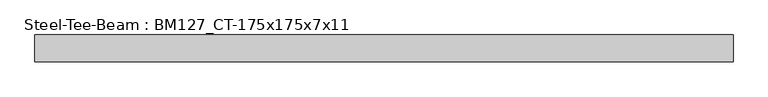
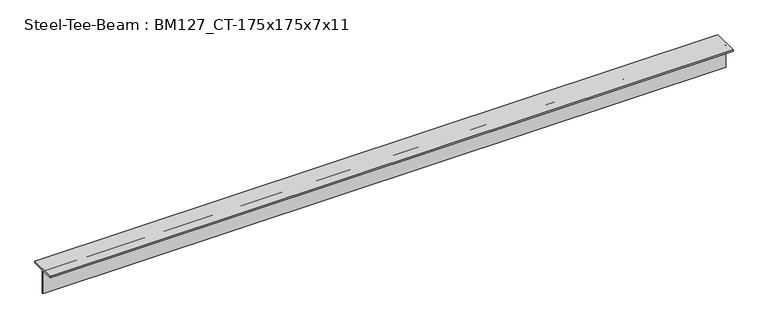
"""IFC4 building model written with IfcOpenShell, lengths in millimetres: beam geometry, Steel-Tee-Beam : BM127_CT-175x175x7x11."""

import ifcopenshell
import ifcopenshell.guid

model = None  # the IFC model being written
_history = None  # IfcOwnerHistory: only IFC2X3 demands one
_inside = {}  # id of a spatial element -> (the spatial element, [elements in it])
_under = {}  # id of a project, library or spatial element -> (it, [spatial elements below it])
_declared = {}  # id of a project -> (the project, [libraries it declares])
_typed = {}  # id of a type object -> (the type object, [elements of that type])
_made_of = {}  # id of a material, layer set ... -> (it, [elements and type objects made of it])


def new_model(schema):
    """Start an empty IFC model of exactly this schema.

    Asked for "IFC4X3", IfcOpenShell would pick the latest addendum, in which some entities
    have other attributes; the version numbers below select the first issue.
    IFC2X3 requires an IfcOwnerHistory on every rooted entity: one is made here for all.
    """
    global model, _history
    if schema == "IFC4X3":
        model = ifcopenshell.file(schema_version=(4, 3, 0, 0))
    else:
        model = ifcopenshell.file(schema=schema)
    _inside.clear()
    _under.clear()
    _declared.clear()
    _typed.clear()
    _made_of.clear()
    _history = None
    if model.schema == "IFC2X3":
        org = make("IfcOrganization", Name="unknown")
        user = make(
            "IfcPersonAndOrganization",
            ThePerson=make("IfcPerson", FamilyName="unknown"),
            TheOrganization=org,
        )
        app = make(
            "IfcApplication",
            ApplicationDeveloper=org,
            Version="unknown",
            ApplicationFullName="unknown",
            ApplicationIdentifier="unknown",
        )
        _history = make(
            "IfcOwnerHistory",
            OwningUser=user,
            OwningApplication=app,
            ChangeAction="ADDED",
            CreationDate=0,
        )
    return model


def make(cls, **values):
    """One entity of the class cls with the attributes given. An attribute that is None is left unset."""
    return model.create_entity(
        cls, **{name: value for name, value in values.items() if value is not None}
    )


def rooted(cls, **values):
    """An entity with a GlobalId (a new one), such as an element, a storey or a relation."""
    return make(cls, GlobalId=ifcopenshell.guid.new(), OwnerHistory=_history, **values)


def si_unit(unit_type, name, prefix=None):
    """IfcSIUnit, for example si_unit("LENGTHUNIT", "METRE", prefix="MILLI")."""
    return make("IfcSIUnit", UnitType=unit_type, Prefix=prefix, Name=name)


def assignment(units):
    """IfcUnitAssignment: the units of a project."""
    return None if units is None else make("IfcUnitAssignment", Units=units)


def point(xyz):
    """IfcCartesianPoint."""
    return None if xyz is None else make("IfcCartesianPoint", Coordinates=xyz)


def direction(xyz):
    """IfcDirection."""
    return None if xyz is None else make("IfcDirection", DirectionRatios=xyz)


def frame(location, z_axis=None, x_axis=None):
    """IfcAxis2Placement3D, a coordinate frame: its origin and axes. An axis left out is left unset."""
    return make(
        "IfcAxis2Placement3D",
        Location=point(location),
        Axis=direction(z_axis),
        RefDirection=direction(x_axis),
    )


def frame_2d(location, x_axis=None):
    """IfcAxis2Placement2D, a coordinate frame in the plane: its origin and x axis."""
    return make(
        "IfcAxis2Placement2D", Location=point(location), RefDirection=direction(x_axis)
    )


def origin():
    """The frame at (0, 0, 0) with its axes left unset."""
    return frame((0.0, 0.0, 0.0))


def place(relative_to, where):
    """IfcLocalPlacement: puts the frame where relative to a parent placement (None: the world)."""
    return make(
        "IfcLocalPlacement", PlacementRelTo=relative_to, RelativePlacement=where
    )


def context(
    kind, dimensions, precision=None, world=None, true_north=None, identifier=None
):
    """IfcGeometricRepresentationContext, for example the 3D "Model" context."""
    return make(
        "IfcGeometricRepresentationContext",
        ContextIdentifier=identifier,
        ContextType=kind,
        CoordinateSpaceDimension=dimensions,
        Precision=precision,
        WorldCoordinateSystem=world,
        TrueNorth=true_north,
    )


def project(units=None, contexts=None):
    """IfcProject with its units and contexts."""
    return rooted(
        "IfcProject",
        Name="project",
        RepresentationContexts=contexts,
        UnitsInContext=assignment(units),
    )


def spatial(cls, under=None, at=None, **own):
    """A site, building, storey or space (cls), placed at a placement, below another one or the project."""
    s = rooted(cls, ObjectPlacement=at, **own)
    if under is not None:
        _under.setdefault(under.id(), (under, []))[1].append(s)
    return s


def polyline(points):
    """IfcPolyline through the points."""
    return make("IfcPolyline", Points=[point(p) for p in points])


def circle_curve(where, radius):
    """IfcCircle in the frame where."""
    return make("IfcCircle", Position=where, Radius=radius)


def trimmed(basis, trim1, trim2, sense, master):
    """IfcTrimmedCurve: the piece of a basis curve between two trims."""
    return make(
        "IfcTrimmedCurve",
        BasisCurve=basis,
        Trim1=trim1,
        Trim2=trim2,
        SenseAgreement=sense,
        MasterRepresentation=master,
    )


def segment(curve, same_sense, transition):
    """IfcCompositeCurveSegment."""
    return make(
        "IfcCompositeCurveSegment",
        Transition=transition,
        SameSense=same_sense,
        ParentCurve=curve,
    )


def composite_curve(segments, self_intersect=None):
    """IfcCompositeCurve: segments joined end to end."""
    return make("IfcCompositeCurve", Segments=segments, SelfIntersect=self_intersect)


def outline(outer, holes=None, kind="AREA"):
    """IfcArbitraryClosedProfileDef: a profile drawn as a closed curve; with holes, ...WithVoids."""
    if holes is None:
        return make("IfcArbitraryClosedProfileDef", ProfileType=kind, OuterCurve=outer)
    return make(
        "IfcArbitraryProfileDefWithVoids",
        ProfileType=kind,
        OuterCurve=outer,
        InnerCurves=holes,
    )


def extrude(swept, where, along, depth):
    """IfcExtrudedAreaSolid: the profile swept, set in the frame where, extruded along a direction by depth."""
    return make(
        "IfcExtrudedAreaSolid",
        SweptArea=swept,
        Position=where,
        ExtrudedDirection=direction(along),
        Depth=depth,
    )


def shape(context_of_items, identifier, shape_type, items):
    """IfcShapeRepresentation: the items that make up one representation, for example the "Body"."""
    return make(
        "IfcShapeRepresentation",
        ContextOfItems=context_of_items,
        RepresentationIdentifier=identifier,
        RepresentationType=shape_type,
        Items=items,
    )


def source(mapping_origin, context_of_items, identifier, shape_type, items):
    """IfcRepresentationMap: a shape defined once, which mapped items show again and again."""
    return make(
        "IfcRepresentationMap",
        MappingOrigin=mapping_origin,
        MappedRepresentation=shape(context_of_items, identifier, shape_type, items),
    )


def transform(
    local_origin,
    x_axis=None,
    y_axis=None,
    z_axis=None,
    scale=None,
    scale2=None,
    scale3=None,
    uniform=True,
):
    """IfcCartesianTransformationOperator3D, or its non-uniform kind. x_axis, y_axis, z_axis: its Axis1, 2, 3."""
    if uniform:
        return make(
            "IfcCartesianTransformationOperator3D",
            Axis1=direction(x_axis),
            Axis2=direction(y_axis),
            LocalOrigin=point(local_origin),
            Scale=scale,
            Axis3=direction(z_axis),
        )
    return make(
        "IfcCartesianTransformationOperator3DnonUniform",
        Axis1=direction(x_axis),
        Axis2=direction(y_axis),
        LocalOrigin=point(local_origin),
        Scale=scale,
        Axis3=direction(z_axis),
        Scale2=scale2,
        Scale3=scale3,
    )


def mapped(mapping_source, mapping_target):
    """IfcMappedItem: shows the shape of a source again, moved by a transform."""
    return make(
        "IfcMappedItem", MappingSource=mapping_source, MappingTarget=mapping_target
    )


def made_of(thing, what):
    """Note that an element or type object is made of a material, layer set ...; save() writes the relation."""
    if what is not None:
        _made_of.setdefault(what.id(), (what, []))[1].append(thing)
    return thing


def element(
    cls,
    number,
    at=None,
    inside=None,
    cuts=None,
    type_object=None,
    material=None,
    context=None,
    identifier="Body",
    shape_type=None,
    held_by="IfcProductDefinitionShape",
    body=None,
    shapes=None,
    **own,
):
    """One element of the class cls, such as IfcWall. Its Tag is "e" and its number.

    at: its placement. inside: the storey or other place that contains it. cuts: it is an
    opening in that element (IfcRelVoidsElement). A single representation is given by context,
    identifier, shape_type and body (its items); several are given by shapes. held_by: the class
    of the entity that holds the representations. save() writes the other relations.
    """
    e = rooted(cls, Tag="e%d" % number, ObjectPlacement=at, **own)
    if body is not None:
        shapes = [shape(context, identifier, shape_type, body)]
    if shapes is not None:
        e.Representation = make(held_by, Representations=shapes)
    if inside is not None:
        _inside.setdefault(inside.id(), (inside, []))[1].append(e)
    if cuts is not None:
        rooted(
            "IfcRelVoidsElement", RelatingBuildingElement=cuts, RelatedOpeningElement=e
        )
    if type_object is not None:
        _typed.setdefault(type_object.id(), (type_object, []))[1].append(e)
    return made_of(e, material)


def aggregate(whole, parts):
    """IfcRelAggregates: a whole, such as a stair, and the parts it consists of."""
    return rooted("IfcRelAggregates", RelatingObject=whole, RelatedObjects=parts)


def save(model, path):
    """Write the relations noted so far, then the file.

    IfcRelAggregates (storeys below a building ...), IfcRelContainedInSpatialStructure (elements
    in a storey), IfcRelDefinesByType, IfcRelAssociatesMaterial and IfcRelDeclares: one each for
    every whole, place, type object, material and project.
    """
    for whole, parts in _under.values():
        aggregate(whole, parts)
    for where, things in _inside.values():
        rooted(
            "IfcRelContainedInSpatialStructure",
            RelatedElements=things,
            RelatingStructure=where,
        )
    for kind, things in _typed.values():
        rooted("IfcRelDefinesByType", RelatedObjects=things, RelatingType=kind)
    for what, things in _made_of.values():
        rooted("IfcRelAssociatesMaterial", RelatedObjects=things, RelatingMaterial=what)
    for by, libraries in _declared.values():
        rooted("IfcRelDeclares", RelatingContext=by, RelatedDefinitions=libraries)
    model.write(path)


def steel_tee_beam_bm127_ct_175x175x7x11_df70e9a8(model_context):
    return source(origin(), model_context, "Body", "SweptSolid", [
        extrude(outline(composite_curve([segment(polyline([(87.5, 87.5), (87.5, 76.5), (17.5, 76.5)]), True, "CONTINUOUS"), segment(trimmed(circle_curve(frame_2d((17.5, 62.5)), 14.0), [point((17.5, 76.5))], [point((3.5, 62.5))], True, "CARTESIAN"), True, "CONTINUOUS"), segment(polyline([(3.5, 62.5), (3.5, -87.5), (-3.5, -87.5), (-3.5, 62.5)]), True, "CONTINUOUS"), segment(trimmed(circle_curve(frame_2d((-17.5, 62.5)), 14.0), [point((-3.5, 62.5))], [point((-17.5, 76.5))], True, "CARTESIAN"), True, "CONTINUOUS"), segment(polyline([(-17.5, 76.5), (-87.5, 76.5), (-87.5, 87.5), (87.5, 87.5)]), True, "CONTINUOUS")], self_intersect=False)), frame((-2375.7579713, 0.0, 0.0), z_axis=(1.0, 0.0, 0.0), x_axis=(0.0, 1.0, 0.0)), (0.0, 0.0, 1.0), 4573.2110535),
    ])


if __name__ == "__main__":
    model = new_model("IFC4")
    model_context = context("Model", 3, world=origin())
    ifc_project = project(units=[si_unit("LENGTHUNIT", "METRE", prefix="MILLI")], contexts=[model_context])
    site = spatial("IfcSite", under=ifc_project)
    building = spatial("IfcBuilding", under=site)
    placement = place(None, origin())
    steel_tee_beam_bm127_ct_175x175x7x11_shape = steel_tee_beam_bm127_ct_175x175x7x11_df70e9a8(model_context)
    element("IfcBeam", 1, ObjectType="Steel-Tee-Beam : BM127_CT-175x175x7x11", at=placement, inside=building, context=model_context, shape_type="MappedRepresentation", body=[
        mapped(steel_tee_beam_bm127_ct_175x175x7x11_shape, transform((0.0, 0.0, 0.0), x_axis=(1.0, 0.0, 0.0), y_axis=(0.0, 1.0, 0.0), z_axis=(0.0, 0.0, 1.0))),
    ])
    save(model, "model.ifc")

# Revit data of these elements
# Type "Steel-Tee-Beam : BM127_CT-175x175x7x11"
#   Surface Area = 0.00 m²/m
#   Section Area = 31.57 cm²
#   Mass per Unit Length = 24.80 kg/m
#   Length [instance default] = 1524 mm
#   bf = 175 mm
#   d = 175 mm
#   k = 25 mm
#   kr = 14 mm
#   tf = 11 mm
#   tw = 7 mm
#   hec_material4 [instance default] = none
#   hec_material3 [instance default] = none
#   hec_material2 [instance default] = none
#   hec_material1 [instance default] = none
#   Structural Material [instance default] = Steel, 45-345
#   Assembly Code = ""
# Element 1 (IfcBeam, "Steel-Tee-Beam : BM127_CT-175x175x7x11")
#   hec_material3 = F01AC000-00002_Building/Shelter Fire Proofing Work_Intumescent Coating Type_1 hr. rating (UL 1709))
#   hec_material2 = S01AA010-00002_Main Steel Structure Fabrication Work_Shelter/Building_Steel Painting/Coating_for Fireproofed Steel Surface, Surface Preparation & Primer Coat
#   hec_material1 = S03AA029-00001_Main Steel Structure Erection Work_Shelter/Building_Light Steel
#   Structural Material = S01AA003-00001_Main Steel Structure Fabrication Work_Shelter/Building_Light Steel - Standard
#   Materials on its faces: "S01AA003-00001_Main Steel Structure Fabrication Work_Shelter/Building_Light Steel - Standard"
# Materials
#   "Steel, 45-345": class "Metal", colour RGB 189 187 185, transparency 0, Description = "Steel 345 MPa", Cost = 0
#   "S01AA003-00001_Main Steel Structure Fabrication Work_Shelter/Building_Light Steel - Standard": class "Metal", colour RGB 120 120 120, transparency 0, Comments = "(30KG/M>Weight)", Description = "Structural steel 50ksi", W00) Work Master Code = "S01AA003-00001", W01) Work Master_Lv1 = "Main Steel Structure Fabrication Work", W02) Work Master_Lv2 = "Shelter/Building", W03) Work Master_Spec.1 = "Light Steel - Standard (30KG/M>Weight)", Cost = 0
#   "F01AC000-00002_Building/Shelter Fire Proofing Work_Intumescent Coating Type_1 hr. rating (UL 1709))": class "Metal", colour RGB 255 128 128, transparency 0, Description = "Paint finished steel", W00) Work Master Code = "F01AC000-00002", W01) Work Master_Lv1 = "Building/Shelter Fire Proofing Work", W02) Work Master_Lv2 = "Intumescent Coating Type", W03) Work Master_Spec.1 = "1 hr. rating (UL 1709)", Cost = 0
#   "S01AA010-00002_Main Steel Structure Fabrication Work_Shelter/Building_Steel Painting/Coating_for Fireproofed Steel Surface, Surface Preparation & Primer Coat": class "Metal", colour RGB 120 120 120, transparency 0, Description = "Paint finished steel", W00) Work Master Code = "SS01AA010-00002", W01) Work Master_Lv1 = "Main Steel Structure Fabrication Work", W02) Work Master_Lv2 = "Shelter/Building", W03) Work Master_Spec.1 = "Steel Painting/Coating", W04) Work Master_Spec.2 = "for Fireproofed Steel Surface, Surface Preparation & Primer Coat", Cost = 0
#   "S03AA029-00001_Main Steel Structure Erection Work_Shelter/Building_Light Steel": class "Metal", colour RGB 120 120 120, transparency 0, Comments = "(30KG/M>Weight)", Description = "Structural steel 50ksi", W00) Work Master Code = "S03AA029-00001", W01) Work Master_Lv1 = "Main Steel Structure Erection Work", W02) Work Master_Lv2 = "Shelter/Building", W03) Work Master_Spec.1 = "Light Steel (30KG/M>Weight)", Cost = 0
